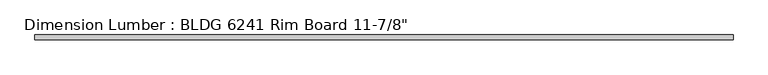
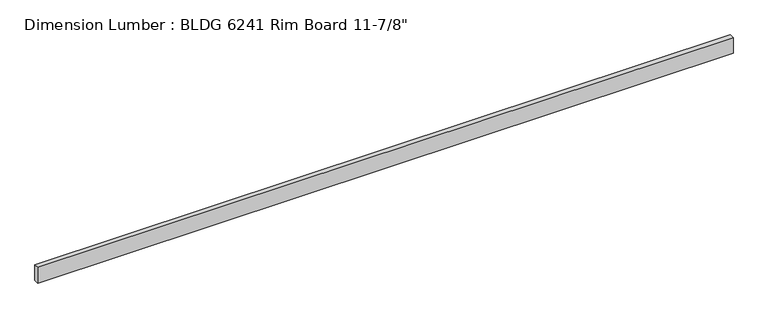
"""IFC4 building model written with IfcOpenShell, lengths in millimetres: beam geometry."""

from ifc_helpers import new_model, si_unit, frame, origin, place, context, project, spatial, polyline, outline, extrude, source, transform, mapped, element, save


def beam_06e53553(model_context):
    return source(origin(), model_context, "Body", "SweptSolid", [
        extrude(outline(polyline([(6332.8098719, 44.45), (6332.8098719, -44.45), (-6377.2598719, -44.45), (-6377.2598719, 44.45), (6332.8098719, 44.45)])), frame((0.0, 0.0, -150.8125), z_axis=(0.0, 0.0, 1.0), x_axis=(1.0, 0.0, 0.0)), (0.0, 0.0, 1.0), 301.625),
    ])


if __name__ == "__main__":
    model = new_model("IFC4")
    model_context = context("Model", 3, world=origin())
    ifc_project = project(units=[si_unit("LENGTHUNIT", "METRE", prefix="MILLI")], contexts=[model_context])
    site = spatial("IfcSite", under=ifc_project)
    building = spatial("IfcBuilding", under=site)
    placement = place(None, origin())
    beam_shape = beam_06e53553(model_context)
    element("IfcBeam", 1, ObjectType="Dimension Lumber : BLDG 6241 Rim Board 11-7/8\"", at=placement, inside=building, context=model_context, shape_type="MappedRepresentation", body=[
        mapped(beam_shape, transform((0.0, 0.0, 0.0), x_axis=(1.0, 0.0, 0.0), y_axis=(0.0, 1.0, 0.0), z_axis=(0.0, 0.0, 1.0))),
    ])
    save(model, "model.ifc")

# Revit data of these elements
# Type "Dimension Lumber : BLDG 6241 Rim Board 11-7/8\""
#   Assembly Code = "B10"
#   A = 0.273472 SF
#   Length [instance default] = 5' - 0"
#   b = 0' - 3 1/2"
#   d = 0' - 11 7/8"
#   Structural Material [instance default] = Softwood, Lumber
# Element 1 (IfcBeam, "Dimension Lumber : BLDG 6241 Rim Board 11-7/8\"")
#   Materials on its faces: "Softwood, Lumber"
# Materials
#   "Softwood, Lumber": class "Wood", colour RGB 223 192 134, transparency 0, Description = "Pinus Echinata", Cost = 0
